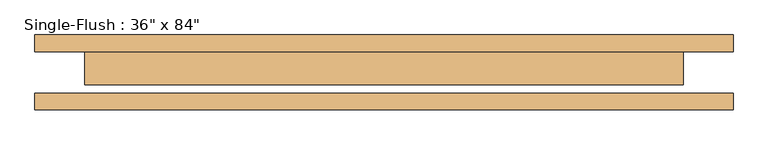
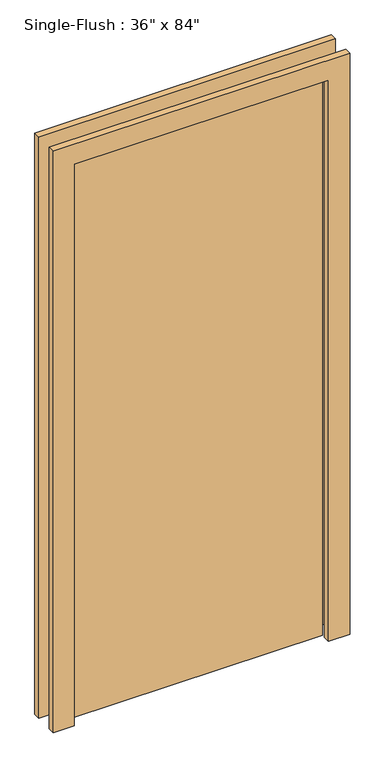
"""IFC4 building model written with IfcOpenShell, lengths in millimetres: door geometry."""

from ifc_helpers import new_model, si_unit, frame, origin, origin_with_axes, place, context, project, spatial, polyline, outline, extrude, source, transform, mapped, element, save


def door_5bbd86ef(model_context):
    return source(origin(), model_context, "Body", "SweptSolid", [
        extrude(outline(polyline([(2209.8, -533.4), (0.0, -533.4), (0.0, -457.2), (2133.6, -457.2), (2133.6, 457.2), (0.0, 457.2), (0.0, 533.4), (2209.8, 533.4), (2209.8, -533.4)])), frame((0.0, 31.75, 0.0), z_axis=(0.0, 1.0, 0.0), x_axis=(0.0, 0.0, 1.0)), (0.0, 0.0, 1.0), 25.4),
        extrude(outline(polyline([(2209.8, 533.4), (2209.8, -533.4), (0.0, -533.4), (0.0, -457.2), (2133.6, -457.2), (2133.6, 457.2), (0.0, 457.2), (0.0, 533.4), (2209.8, 533.4)])), frame((0.0, -57.15, 0.0), z_axis=(0.0, 1.0, 0.0), x_axis=(0.0, 0.0, 1.0)), (0.0, 0.0, 1.0), 25.4),
        extrude(outline(polyline([(457.2, -19.05), (-457.2, -19.05), (-457.2, 31.75), (457.2, 31.75), (457.2, -19.05)])), origin_with_axes(), (0.0, 0.0, 1.0), 2133.6),
    ])


if __name__ == "__main__":
    model = new_model("IFC4")
    model_context = context("Model", 3, world=origin())
    ifc_project = project(units=[si_unit("LENGTHUNIT", "METRE", prefix="MILLI")], contexts=[model_context])
    site = spatial("IfcSite", under=ifc_project)
    building = spatial("IfcBuilding", under=site)
    placement = place(None, origin())
    door_shape = door_5bbd86ef(model_context)
    element("IfcDoor", 1, ObjectType="Single-Flush : 36\" x 84\"", at=placement, inside=building, context=model_context, shape_type="MappedRepresentation", body=[
        mapped(door_shape, transform((0.0, 0.0, 0.0), x_axis=(1.0, 0.0, 0.0), y_axis=(0.0, 1.0, 0.0), z_axis=(0.0, 0.0, 1.0))),
    ])
    save(model, "model.ifc")

# Revit data of these elements
# Type "Single-Flush : 36\" x 84\""
#   Type Mark = "1"
#   Construction Type Id = "MDOOR"
#   Assembly Code = "C1020"
#   Analytic Construction = "Metal"
#   Thickness = 0' - 2"
#   Heat Transfer Coefficient (U) = 0.651978 BTU/(h·ft²·°F)
#   Height = 7' - 0"
#   Trim Projection Ext = 0' - 1"
#   Trim Projection Int = 0' - 1"
#   Trim Width = 0' - 3"
#   Width = 3' - 0"
#   Define Thermal Properties by = 1
#   Define Thermal Properties by = 1
#   Door Material = Door - Panel
#   Frame Material = Door - Frame
#   Visual Light Transmittance = 0
#   Solar Heat Gain Coefficient = 0
#   Function = (empty or 0)
#   Wall Closure = (empty or 0)
# Element 1 (IfcDoor, "Single-Flush : 36\" x 84\"")
#   Materials on its faces: "Door - Frame", "Door - Panel"
# Materials
#   "Door - Panel": class "Wood", colour RGB 210 159 95, transparency 0, Cost = 0
#   "Door - Frame": class "Miscellaneous", colour RGB 118 70 51, transparency 0, Cost = 0
